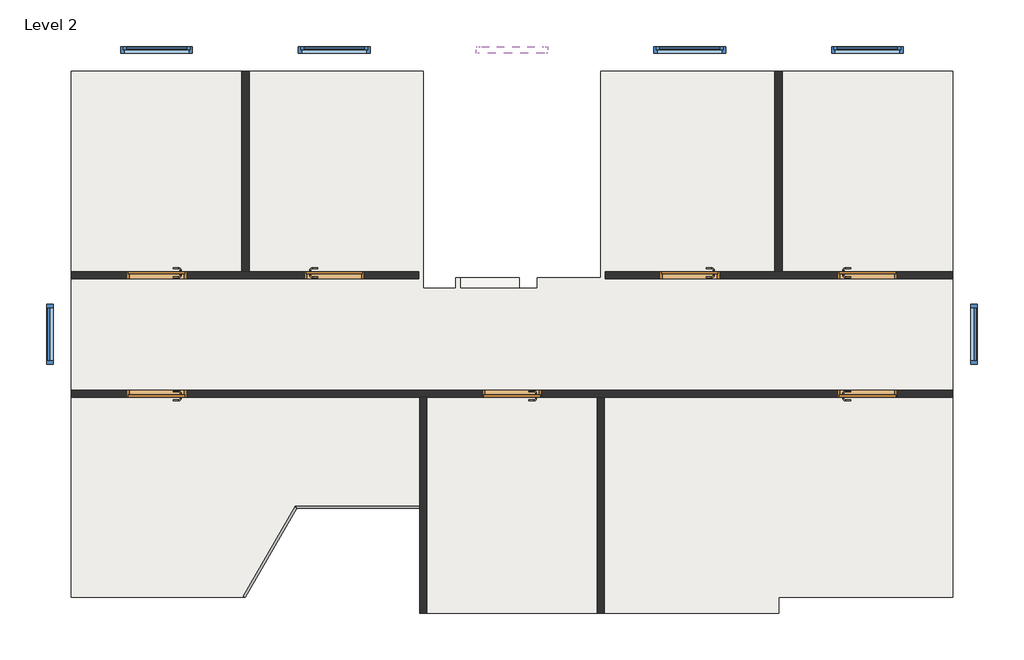
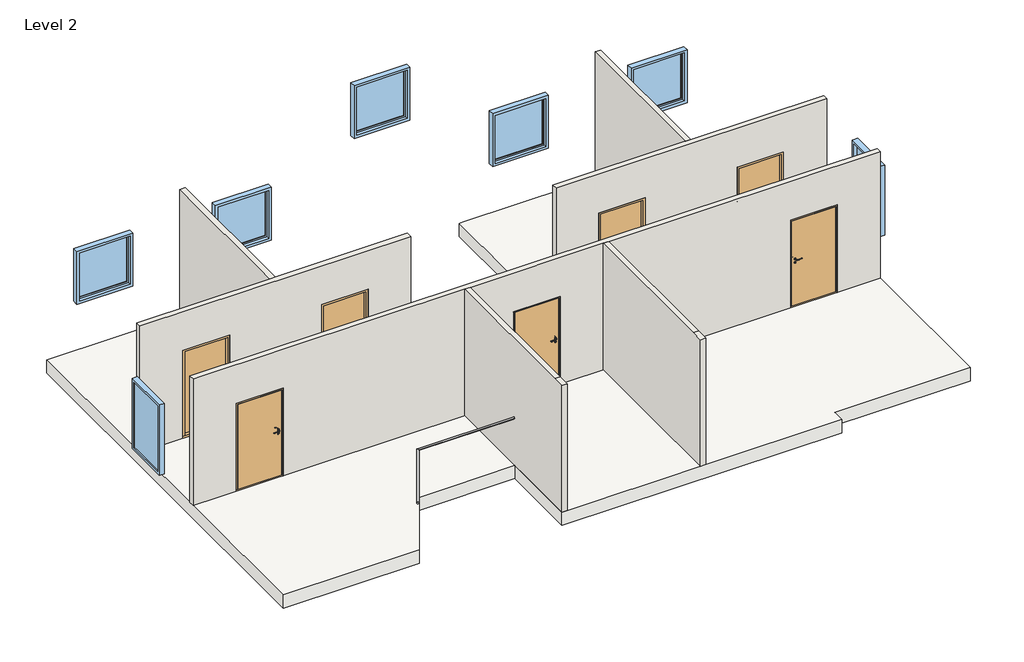
# One storey: 7 doors, 7 walls, 7 windows, 1 railing, 1 slab.
# Revit data of these elements (continued)
# Type "Int. Single-Flush : 10x20M" (continued)
#   Creator Build [instance default] = "2017.0801.0"
#   Analytic Construction = "<None>"
#   length#5 = 1012 mm
#   length#3 = 42 mm
#   length#2b = 12 mm
#   length#2a = 0 mm
#   length#2 = 0 mm
#   length#1a = 12 mm
#   length#1 = 0 mm
#   length#4 = 30 mm
#   Thickness = 40 mm
#   Seal Width = 12 mm
#   Rough Width = 1012 mm
#   Rough Height = 2012 mm
#   Rabbet Depth = 40 mm
#   Interior Distance [instance default] = 0 mm
#   Height = 1988 mm
#   Width = 988 mm
#   Handle From Side = 100 mm
#   Handle From Bottom = 1090 mm
#   Exterior Direction [instance default] = 0.00°
#   Case Depth [instance default] = 200 mm
#   Case Width = 30 mm
#   Rabbet Width = 12 mm
#   Exterior Distance [instance default] = 0 mm
#   Bottom Seal = 12 mm
#   Threshold = yes
#   Sealing = no
#   Hinging = yes
#   Wall Closure = 1
#   Door Panel = no
#   Panel = none
#   Handle Finish = none
#   Handle = element 510752
#   Case/Transom = none
#   Function = (empty or 0)
#   Assembly Code = ""
# Type "Sketch 1100mm"
#   built-in parameter 1008612 = 0.019685 (stored number, unit not read)
#   built-in parameter 1008611 = 0.019685 (stored number, unit not read)
#   built-in parameter 1008609 = 0.902231 (stored number, unit not read)
#   built-in parameter 1008604 = 0.19685 (stored number, unit not read)
#   built-in parameter 1008603 = 0.164042 (stored number, unit not read)
#   Railing Height = 1100 mm
#   built-in parameter 1008632 = 1
#   built-in parameter 1008630 = 2
#   built-in parameter 1008610 = 2
# Type "Suspended - 300mm LW Concrete / Wood Planks"
#   Function = 0
#   Layers, outside or top first: 22 mm "Wood Planks" (function 4); 0 mm "Flooring Underlay" (function 100); 58 mm "Concrete, Broom Finish" (function 2); 220 mm "Concrete, Lightweight Precast" (function 1)
# Type "Interior - 120mm Drywall (25/70/25)"
#   Layers, outside or top first: 25 mm "Gypsum Plasterboard" (function 5); 70 mm "Batt insulation" (function 2); 25 mm "Gypsum Plasterboard" (function 5)
# Type "Interior - 120mm LW Concrete"
#   Layers, outside or top first: 120 mm "Concrete, Lightweight Precast" (function 1)
# Type "Fixed : 10x16M"
#   Type Mark = "59"
#   Creator Organization [instance default] = "© Danish Educational Content"
#   Creator Name [instance default] = "© Erik Falck Jørgensen"
#   Creator Build [instance default] = "2017.0801.0"
#   Analytic Construction = "<None>"
#   length#5 = -22 mm
#   length#4 = -50 mm
#   length#3 = 100 mm
#   length#2 = 57 mm
#   length#1 = 0 mm
#   Seal Width = 12 mm
#   Rough Width = 1012 mm
#   Rough Height = 1612 mm
#   Rebate Depth = 50 mm
#   Height = 1588 mm
#   Glass Thickness = 28 mm
#   Exterior Direction [instance default] = 0.00°
#   Default Sill Height = 800 mm
#   Width = 988 mm
#   Case Width = 45 mm
#   Case Depth = 115 mm
#   Sealing = no
#   Wall Closure = 1
#   Above Cutplane [instance default] = no
#   Wall Surface = none
#   Sill Plate = none
#   Glass = none
#   Embrasure = none
#   Case/Transom = none
#   Assembly Code = ""
# Type "Single-Light : 12x12M"
#   Type Mark = "39"
#   Creator Organization [instance default] = "© Danish Educational Content"
#   Creator Name [instance default] = "© Erik Falck Jørgensen"
#   Creator Build [instance default] = "2017.0801.0"
#   Analytic Construction = "<None>"
#   length#5 = -36 mm
#   length#4 = -14 mm
#   length#3 = 120 mm
#   length#2 = 57 mm
#   length#1 = 0 mm
#   Seal Width = 12 mm
#   Rough Width = 1212 mm
#   Rough Height = 1212 mm
#   Rebate Depth = 50 mm
#   Rabbet Width = 15 mm
#   Rabbet Depth = 50 mm
#   Height = 1188 mm
#   Glass Thickness = 22 mm
#   Frame Width = 50 mm
#   Frame Depth = 50 mm
#   Exterior Direction [instance default] = 0.00°
#   Case Depth = 115 mm
#   Case Width = 45 mm
#   Default Sill Height = 800 mm
#   Width = 1188 mm
#   Sealing = no
#   Hinging = yes
#   Wall Closure = 1
#   Above Cutplane [instance default] = no
#   Wall Surface = none
#   Sill Plate = none
#   Glass = none
#   Frame/Mullion = none
#   Embrasure = none
#   Case/Transom = none
# Elements 1, 2, 3, 4, 5, 6, 7 (IfcDoor, "Int. Single-Flush : 10x20M")
#   Hinge Side = ""
#   Creator Organization = "© Danish Educational Content"
#   Creator Name = "© Erik Falck Jørgensen"
#   Creator Build = "2017.0801.0"
#   Interior Distance = 0 mm
#   Exterior Distance = 0 mm
#   Exterior Direction = 0.00°
#   Phase Created = New Construction
#   Materials on its faces: "Stainless Steel, Polished", "Default Frame/Mullion (Interior/Exterior)", "Default Door Panel (Exterior/Interior)"
# Element 8 (IfcRailing, "Sketch 1100mm")
#   Phase Created = New Construction
#   Materials on its faces: "Default Railings (Interior/Exterior)"
# Element 9 (IfcSlab, "Suspended - 300mm LW Concrete / Wood Planks")
#   built-in parameter 1001955 = 1.5708 (stored number, unit not read)
#   Height Offset From Level = 0 mm
#   Phase Created = New Construction
#   Materials on its faces: "Concrete, Lightweight Precast", "Wood Planks"
# Elements 10, 11, 12, 13 (IfcWall, "Interior - 120mm Drywall (25/70/25)")
#   Top Offset = 0 mm
#   Base Offset = 0 mm
#   wall height = 2900 mm
#   Phase Created = New Construction
#   Base Constraint = Level 2
#   Top Constraint = Level 3
#   Materials on its faces: "Default Wall", "Gypsum Plasterboard"
# Elements 14, 15, 16 (IfcWall, "Interior - 120mm LW Concrete")
#   Top Offset = 0 mm
#   Base Offset = 0 mm
#   wall height = 2900 mm
#   Phase Created = New Construction
#   Base Constraint = Level 2
#   Top Constraint = Level 3
#   Materials on its faces: "Concrete, Lightweight Precast"
# Element 17 (IfcWindow, "Fixed : 10x16M")
#   Mark = "24"
#   Creator Organization = "© Danish Educational Content"
#   Creator Name = "© Erik Falck Jørgensen"
#   Creator Build = "2017.0801.0"
#   Exterior Direction = 0.00°
#   Above Cutplane = no
#   Phase Created = New Construction
#   Materials on its faces: "Default Frame/Mullion (Interior/Exterior)", "Glass"
# Element 18 (IfcWindow, "Fixed : 10x16M")
#   Mark = "25"
#   Creator Organization = "© Danish Educational Content"
#   Creator Name = "© Erik Falck Jørgensen"
#   Creator Build = "2017.0801.0"
#   Exterior Direction = 0.00°
#   Above Cutplane = no
#   Phase Created = New Construction
#   Materials on its faces: "Default Frame/Mullion (Interior/Exterior)", "Glass"
# Element 19 (IfcWindow, "Single-Light : 12x12M")
#   Mark = "28"
#   Creator Organization = "© Danish Educational Content"
#   Creator Name = "© Erik Falck Jørgensen"
#   Creator Build = "2017.0801.0"
#   Exterior Direction = 0.00°
#   Above Cutplane = no
#   Phase Created = New Construction
#   Materials on its faces: "Default Frame/Mullion (Interior/Exterior)", "Glass"
# Element 20 (IfcWindow, "Single-Light : 12x12M")
#   Mark = "29"
#   Creator Organization = "© Danish Educational Content"
#   Creator Name = "© Erik Falck Jørgensen"
#   Creator Build = "2017.0801.0"
#   Exterior Direction = 0.00°
#   Above Cutplane = no
#   Phase Created = New Construction
#   Materials on its faces: "Default Frame/Mullion (Interior/Exterior)", "Glass"
# Element 21 (IfcWindow, "Single-Light : 12x12M")
#   Mark = "30"
#   Creator Organization = "© Danish Educational Content"
#   Creator Name = "© Erik Falck Jørgensen"
#   Creator Build = "2017.0801.0"
#   Exterior Direction = 0.00°
#   Above Cutplane = no
#   Phase Created = New Construction
#   Materials on its faces: "Default Frame/Mullion (Interior/Exterior)", "Glass"
# Element 22 (IfcWindow, "Single-Light : 12x12M")
#   Mark = "31"
#   Creator Organization = "© Danish Educational Content"
#   Creator Name = "© Erik Falck Jørgensen"
#   Creator Build = "2017.0801.0"
#   Exterior Direction = 0.00°
#   Above Cutplane = no
#   Phase Created = New Construction
#   Materials on its faces: "Default Frame/Mullion (Interior/Exterior)", "Glass"
# Element 23 (IfcWindow, "Single-Light : 12x12M")
#   Mark = "32"
#   Creator Organization = "© Danish Educational Content"
#   Creator Name = "© Erik Falck Jørgensen"
#   Creator Build = "2017.0801.0"
#   Exterior Direction = 0.00°
#   Above Cutplane = no
#   Phase Created = New Construction
#   Materials on its faces: "Default Frame/Mullion (Interior/Exterior)", "Glass"
# Materials
#   "Wood Planks": class "Wood", colour RGB 117 91 64, transparency 0, Description = "Generisk trægulv", Cost = 0
#   "Flooring Underlay": class "Generic", colour RGB 255 0 0, transparency 0, Description = "Gulvunderlag", Cost = 0
#   "Concrete, Broom Finish": class "Concrete", colour RGB 80 80 80, transparency 0, Description = "Beton - afkostet overflade", Cost = 0
#   "Concrete, Lightweight Precast": class "Concrete", colour RGB 180 180 180, transparency 0, Description = "Præfabrikeret letbeton", Cost = 0
#   "Gypsum Plasterboard": class "Generic", colour RGB 180 180 180, transparency 0, Description = "Alm. indvendige gipsplader", Cost = 0
#   "Batt insulation": class "Insulation", colour RGB 255 240 100, transparency 0, Description = "Generisk blød isolering", Cost = 0
#   "Stainless Steel, Polished": class "Metal", colour RGB 180 180 180, transparency 0, Description = "Rustfri stål, poleret", Cost = 0
#   "Default Frame/Mullion (Interior/Exterior)": class "Generic", colour RGB 205 205 205, transparency 0, Description = "Udefineret karm/ramme materiale", Cost = 0
#   "Default Door Panel (Exterior/Interior)": class "Generic", colour RGB 205 205 205, transparency 0, Description = "Udefineret dørplade materiale", Cost = 0
#   "Default Railings (Interior/Exterior)": class "Generic", colour RGB 205 205 205, transparency 0, Description = "Udefineret gelænder materiale", Cost = 0
#   "Default Wall": class "Generic", colour RGB 180 180 180, transparency 0, Description = "Udefineret væg materiale", Cost = 0
#   "Glass": class "Glass", colour RGB 180 200 255, transparency 0.75, Description = "Generisk glas", Cost = 0
